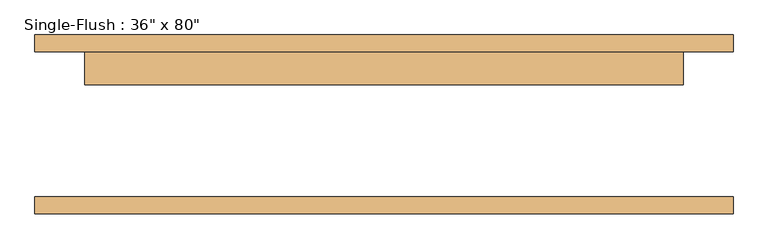
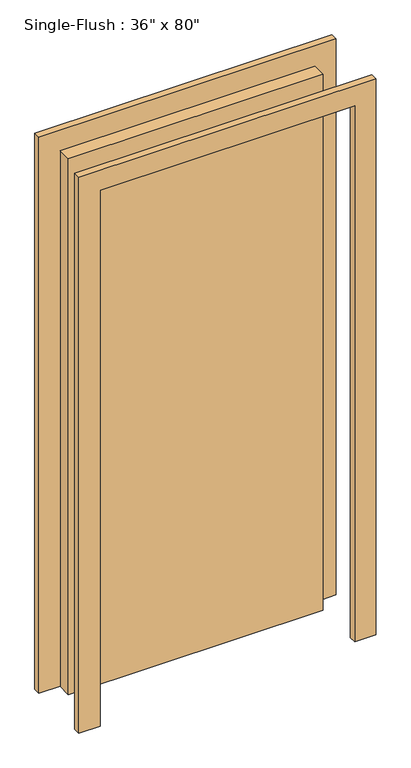
"""IFC4 building model written with IfcOpenShell, lengths in millimetres: door geometry."""

from ifc_helpers import new_model, si_unit, frame, origin, origin_with_axes, place, context, project, spatial, polyline, outline, extrude, source, transform, mapped, element, save


def door_521908aa(model_context):
    return source(origin(), model_context, "Body", "SweptSolid", [
        extrude(outline(polyline([(2108.2, -533.4), (0.0, -533.4), (0.0, -457.2), (2032.0, -457.2), (2032.0, 457.2), (0.0, 457.2), (0.0, 533.4), (2108.2, 533.4), (2108.2, -533.4)])), frame((0.0, 111.125, 0.0), z_axis=(0.0, 1.0, 0.0), x_axis=(0.0, 0.0, 1.0)), (0.0, 0.0, 1.0), 25.4),
        extrude(outline(polyline([(2108.2, 533.4), (2108.2, -533.4), (0.0, -533.4), (0.0, -457.2), (2032.0, -457.2), (2032.0, 457.2), (0.0, 457.2), (0.0, 533.4), (2108.2, 533.4)])), frame((0.0, -136.525, 0.0), z_axis=(0.0, 1.0, 0.0), x_axis=(0.0, 0.0, 1.0)), (0.0, 0.0, 1.0), 25.4),
        extrude(outline(polyline([(457.2, 60.325), (-457.2, 60.325), (-457.2, 111.125), (457.2, 111.125), (457.2, 60.325)])), origin_with_axes(), (0.0, 0.0, 1.0), 2032.0),
    ])


if __name__ == "__main__":
    model = new_model("IFC4")
    model_context = context("Model", 3, world=origin())
    ifc_project = project(units=[si_unit("LENGTHUNIT", "METRE", prefix="MILLI")], contexts=[model_context])
    site = spatial("IfcSite", under=ifc_project)
    building = spatial("IfcBuilding", under=site)
    placement = place(None, origin())
    door_shape = door_521908aa(model_context)
    element("IfcDoor", 1, ObjectType="Single-Flush : 36\" x 80\"", at=placement, inside=building, context=model_context, shape_type="MappedRepresentation", body=[
        mapped(door_shape, transform((0.0, 0.0, 0.0), x_axis=(1.0, 0.0, 0.0), y_axis=(0.0, 1.0, 0.0), z_axis=(0.0, 0.0, 1.0))),
    ])
    save(model, "model.ifc")

# Revit data of these elements
# Type "Single-Flush : 36\" x 80\""
#   Type Mark = "13"
#   Construction Type Id = "MDOOR"
#   Assembly Code = "C1020"
#   Analytic Construction = "Metal"
#   Thickness = 0' - 2"
#   Heat Transfer Coefficient (U) = 3.7021 W/(m²·K)
#   Height = 6' - 8"
#   Trim Projection Ext = 0' - 1"
#   Trim Projection Int = 0' - 1"
#   Trim Width = 0' - 3"
#   Width = 3' - 0"
#   Door Material = INTERIOR GRADE ALUMINUM STOREFRONT W/ SAFETY GLAZING
#   Frame Material = INTERIOR GRADE ALUMINUM STOREFRONT W/ SAFETY GLAZING
#   Visual Light Transmittance = 0
#   Solar Heat Gain Coefficient = 0
#   Function = (empty or 0)
#   Wall Closure = (empty or 0)
# Element 1 (IfcDoor, "Single-Flush : 36\" x 80\"")
#   Materials on its faces: "INTERIOR GRADE ALUMINUM STOREFRONT W/ SAFETY GLAZING"
# Materials
#   "INTERIOR GRADE ALUMINUM STOREFRONT W/ SAFETY GLAZING": class "Metal", colour RGB 226 226 226, transparency 0, Description = "Aluminum 6061", Cost = 0
